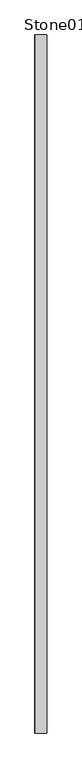
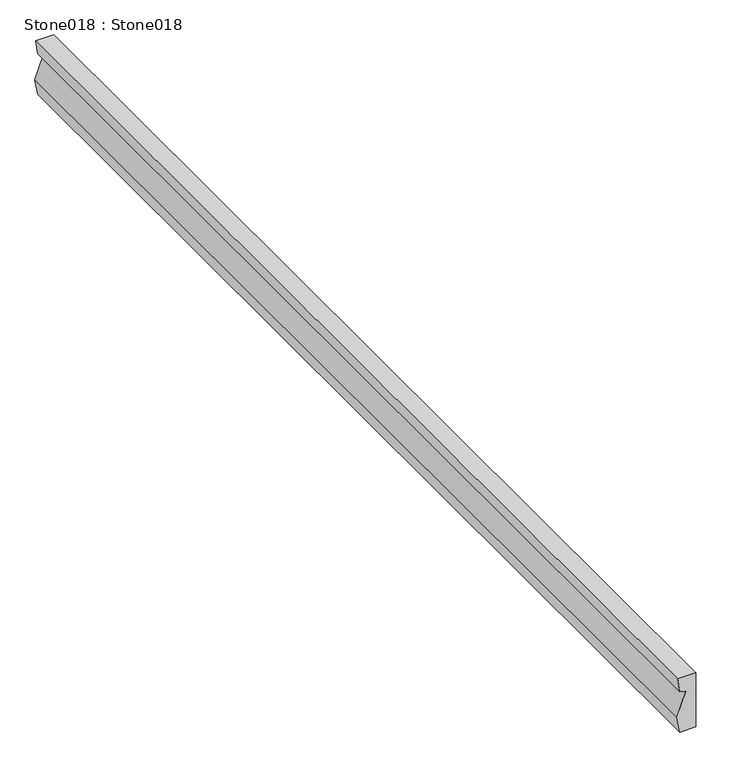
"""IFC4 building model written with IfcOpenShell, lengths in millimetres: proxy geometry, Stone018 : Stone018."""

from ifc_helpers import new_model, si_unit, frame, origin, place, context, project, spatial, polyline, outline, extrude, source, transform, mapped, element, save


def stone018_stone018_3aa1dd09(model_context):
    return source(origin(), model_context, "Body", "SweptSolid", [
        extrude(outline(polyline([(32779.6230469, -10298.3867188), (32753.4921875, -10294.4599609), (32750.2792969, -10284.2871094), (32706.5546875, -10299.8144531), (32676.5371094, -10294.3740234), (32676.5371094, -10266.1494141), (32779.6230469, -10266.1494141), (32779.6230469, -10298.3867188)])), frame((0.0, 7982.1531721, 0.0), z_axis=(0.0, 1.0, 0.0), x_axis=(0.0, 0.0, 1.0)), (0.0, 0.0, 1.0), 2000.0),
    ])


if __name__ == "__main__":
    model = new_model("IFC4")
    model_context = context("Model", 3, world=origin())
    ifc_project = project(units=[si_unit("LENGTHUNIT", "METRE", prefix="MILLI")], contexts=[model_context])
    site = spatial("IfcSite", under=ifc_project)
    building = spatial("IfcBuilding", under=site)
    placement = place(None, origin())
    stone018_stone018_shape = stone018_stone018_3aa1dd09(model_context)
    element("IfcBuildingElementProxy", 1, Name="Stone018 : Stone018", ObjectType="Stone018 : Stone018", at=placement, inside=building, context=model_context, shape_type="MappedRepresentation", body=[
        mapped(stone018_stone018_shape, transform((0.0, 0.0, 0.0), x_axis=(1.0, 0.0, 0.0), y_axis=(0.0, 1.0, 0.0), z_axis=(0.0, 0.0, 1.0))),
    ])
    save(model, "model.ifc")

# Revit data of these elements
# Type "Stone018 : Stone018"
#   NameOverride = "Stone018"
# Element 1 (IfcBuildingElementProxy, "Stone018 : Stone018")
#   Materials on its faces: "SPLIT FACE STONE 1032"
# Materials
#   "SPLIT FACE STONE 1032": class "Unassigned", colour RGB 205 195 181, transparency 0
